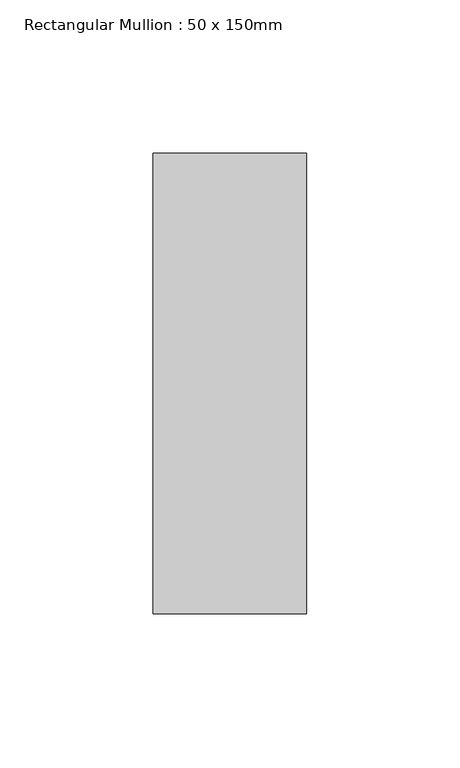
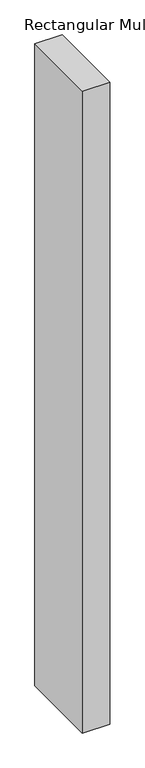
"""IFC4 building model written with IfcOpenShell, lengths in millimetres: member geometry, Rectangular Mullion : 50 x 150mm."""

from ifc_helpers import new_model, si_unit, frame, origin, place, context, project, spatial, polyline, outline, extrude, source, transform, mapped, element, save


def rectangular_mullion_50_x_150mm_23e890aa(model_context):
    return source(origin(), model_context, "Body", "SweptSolid", [
        extrude(outline(polyline([(25.0, 75.0), (25.0, -75.0), (-25.0, -75.0), (-25.0, 75.0), (25.0, 75.0)])), frame((0.0, 0.0, -1240.0000002), z_axis=(0.0, 0.0, 1.0), x_axis=(1.0, 0.0, 0.0)), (0.0, 0.0, 1.0), 1240.0000002),
    ])


if __name__ == "__main__":
    model = new_model("IFC4")
    model_context = context("Model", 3, world=origin())
    ifc_project = project(units=[si_unit("LENGTHUNIT", "METRE", prefix="MILLI")], contexts=[model_context])
    site = spatial("IfcSite", under=ifc_project)
    building = spatial("IfcBuilding", under=site)
    placement = place(None, origin())
    rectangular_mullion_50_x_150mm_shape = rectangular_mullion_50_x_150mm_23e890aa(model_context)
    element("IfcMember", 1, ObjectType="Rectangular Mullion : 50 x 150mm", at=placement, inside=building, context=model_context, shape_type="MappedRepresentation", body=[
        mapped(rectangular_mullion_50_x_150mm_shape, transform((0.0, 0.0, 0.0), x_axis=(1.0, 0.0, 0.0), y_axis=(0.0, 1.0, 0.0), z_axis=(0.0, 0.0, 1.0))),
    ])
    save(model, "model.ifc")

# Revit data of these elements
# Type "Rectangular Mullion : 50 x 150mm"
#   built-in parameter 1007304 = 0.492126 (stored number, unit not read)
#   built-in parameter 1007301 = 0.082021 (stored number, unit not read)
#   built-in parameter 1007300 = 0.082021 (stored number, unit not read)
# Element 1 (IfcMember, "Rectangular Mullion : 50 x 150mm")
#   Materials on its faces: "Aluminium"
# Materials
#   "Aluminium": class "Metal", colour RGB 247 247 247, transparency 0, Description = "Aluminium 6061", Cost = 0
